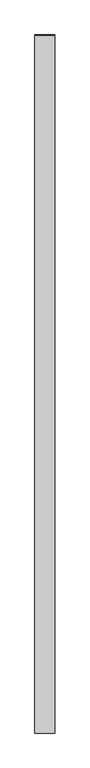
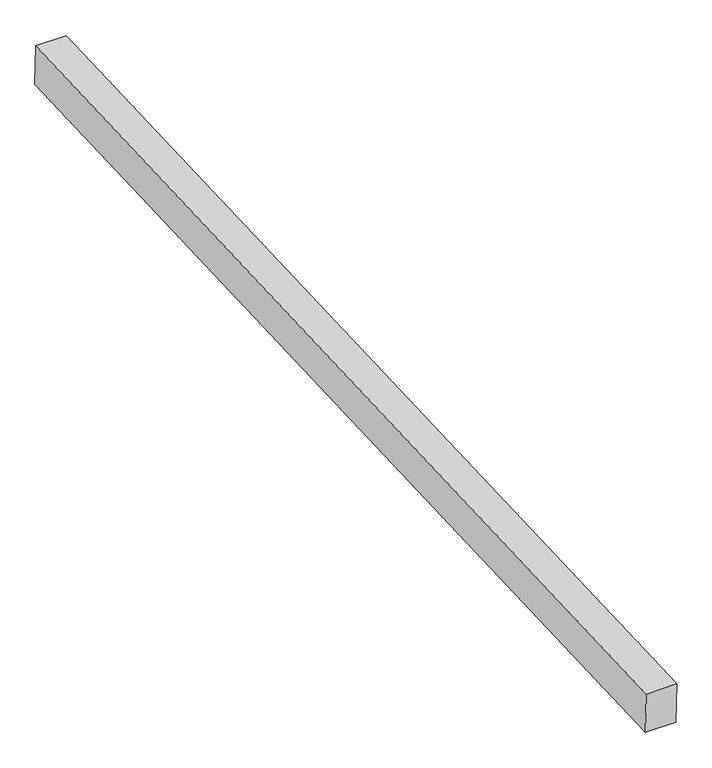
"""IFC4 building model written with IfcOpenShell, lengths in millimetres: proxy geometry, Generic Models 7:Generic Models 1:8:Generic Models 1:8 : Generic Models 7:Generic Models 1:337419:15 : Generic Models 7:Generic Models 1:8:Generic Models 1:8 : Generic Models 7:Generic Models 1:337419:315935."""

from ifc_helpers import new_model, si_unit, frame, origin, place, context, project, spatial, polyline, outline, extrude, source, transform, mapped, element, save


def generic_models_d056ae43(model_context):
    return source(origin(), model_context, "Body", "SweptSolid", [
        extrude(outline(polyline([(-580626.555738, 3844.0209448), (-575753.6328438, 4047.0593987), (-575746.0659221, 3856.7093942), (-580618.6251193, 3653.6860944), (-580626.555738, 3844.0209448)])), frame((591213.961724, 0.0, 0.0), z_axis=(1.0, 0.0, 0.0), x_axis=(0.0, 1.0, 0.0)), (0.0, 0.0, 1.0), 139.7),
    ])


if __name__ == "__main__":
    model = new_model("IFC4")
    model_context = context("Model", 3, world=origin())
    ifc_project = project(units=[si_unit("LENGTHUNIT", "METRE", prefix="MILLI")], contexts=[model_context])
    site = spatial("IfcSite", under=ifc_project)
    building = spatial("IfcBuilding", under=site)
    placement = place(None, origin())
    generic_models_shape = generic_models_d056ae43(model_context)
    element("IfcBuildingElementProxy", 1, Name="Generic Models 7:Generic Models 1:8:Generic Models 1:8 : Generic Models 7:Generic Models 1:337419:15 : Generic Models 7:Generic Models 1:8:Generic Models 1:8 : Generic Models 7:Generic Models 1:337419:315935", ObjectType="Generic Models 7:Generic Models 1:8:Generic Models 1:8 : Generic Models 7:Generic Models 1:337419:15 : Generic Models 7:Generic Models 1:8:Generic Models 1:8 : Generic Models 7:Generic Models 1:337419:315935", at=placement, inside=building, context=model_context, shape_type="MappedRepresentation", body=[
        mapped(generic_models_shape, transform((0.0, 0.0, 0.0), x_axis=(1.0, 0.0, 0.0), y_axis=(0.0, 1.0, 0.0), z_axis=(0.0, 0.0, 1.0))),
    ])
    save(model, "model.ifc")

# Revit data of these elements
# Type "Generic Models 7:Generic Models 1:8:Generic Models 1:8 : Generic Models 7:Generic Models 1:337419:15 : Generic Models 7:Generic Models 1:8:Generic Models 1:8 : Generic Models 7:Generic Models 1:337419:315935"
#   NameOverride = "Generic Models 7:Generic Models 1:8:Generic Models 1:8 : Generic Models 7:Generic Models 1:337419:315935"
#   ObjectTypeOverride = "Generic Models 1:8 : Generic Models 7:Generic Models 1:337419"
#   Reference = "Generic Models 1"
#   Tag = "315935"
# Element 1 (IfcBuildingElementProxy, "Generic Models 7:Generic Models 1:8:Generic Models 1:8 : Generic Models 7:Generic Models 1:337419:15 : Generic Models 7:Generic Models 1:8:Generic Models 1:8 : Generic Models 7:Generic Models 1:337419:315935")
#   Materials on its faces: "5 1/2\" X 7 1/2\" EXTERIOR GRADE GLULAM BEAMS"
# Materials
#   "5 1/2\" X 7 1/2\" EXTERIOR GRADE GLULAM BEAMS": class "Wood", colour RGB 183 134 68, transparency 0, Keynote = "M06181300.01", Description = "Pinus Echinata", Cost = 0
